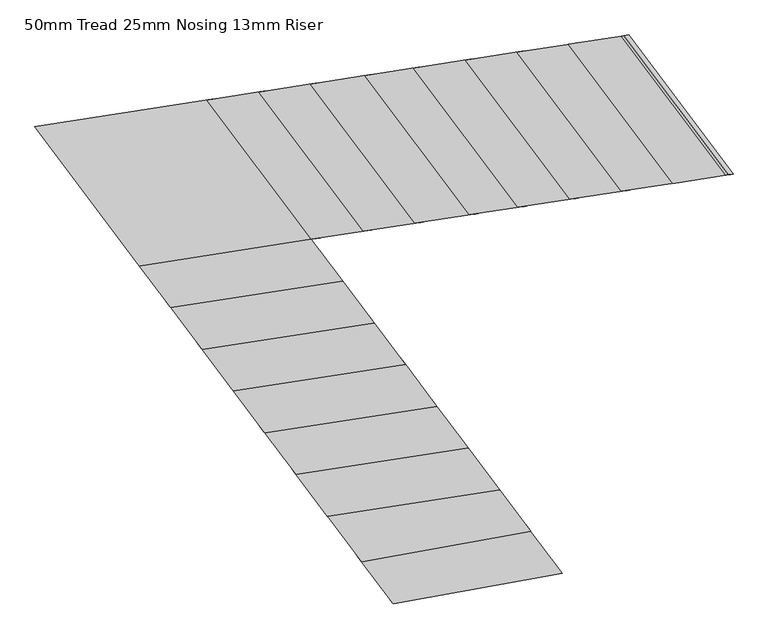
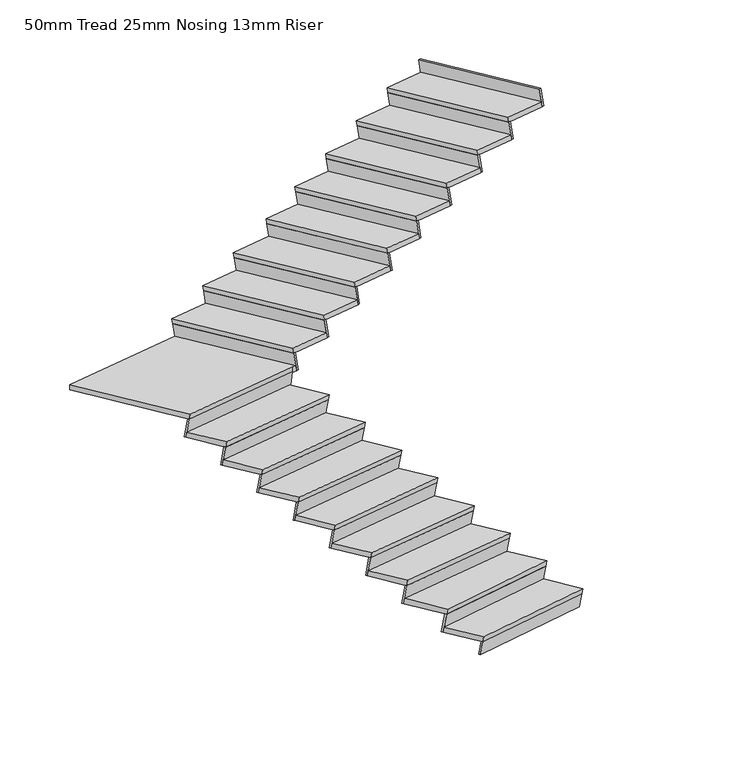
"""IFC4 building model written with IfcOpenShell, lengths in millimetres: stair flight geometry, 50mm Tread 25mm Nosing 13mm Riser."""

from ifc_helpers import new_model, si_unit, origin, place, context, project, spatial, faceted_brep, source, transform, mapped, element, save


def stair_flight_50mm_tread_25mm_nosing_13mm_riser_829bcf17(model_context):
    return source(origin(), model_context, "Body", "Brep", [
        faceted_brep([(80326.693796, 43447.2585725, 17175.0), (80321.8971276, 43453.651768, 17125.0), (79350.3599929, 43278.4852415, 17125.0), (79355.1566613, 43272.092046, 17175.0), (79551.9875613, 43009.747788, 17175.0), (80523.524696, 43184.9143144, 17175.0), (80518.7280276, 43191.3075099, 17125.0), (79547.1908928, 43016.1409835, 17125.0)], [[[0, 1, 2, 3]], [[3, 4, 5, 0]], [[2, 1, 6, 7]], [[4, 3, 2, 7]], [[0, 5, 6, 1]], [[5, 4, 7, 6]]]),
        faceted_brep([(80518.7280276, 43191.3075099, 17125.0), (80506.7363564, 43207.2904987, 17000.0), (80498.2569645, 43218.5921784, 17000.0), (80510.2486356, 43202.6091897, 17125.0), (79547.1908928, 43016.1409835, 17125.0), (79538.7115009, 43027.4426632, 17125.0), (79526.7198298, 43043.425652, 17000.0), (79535.1992217, 43032.1239722, 17000.0)], [[[0, 1, 2, 3]], [[4, 5, 6, 7]], [[1, 0, 4, 7]], [[2, 1, 7, 6]], [[3, 2, 6, 5]], [[0, 3, 5, 4]]]),
        faceted_brep([(80338.6854672, 43431.2755837, 17300.0), (80321.8971276, 43453.651768, 17125.0), (80313.4177356, 43464.9534477, 17125.0), (80330.2060752, 43442.5772635, 17300.0), (79367.1483324, 43256.1090573, 17300.0), (79358.6689405, 43267.410737, 17300.0), (79341.8806009, 43289.7869213, 17125.0), (79350.3599929, 43278.4852415, 17125.0)], [[[0, 1, 2, 3]], [[4, 5, 6, 7]], [[1, 0, 4, 7]], [[2, 1, 7, 6]], [[3, 2, 6, 5]], [[0, 3, 5, 4]]]),
        faceted_brep([(79158.1923254, 43534.614153, 17350.0), (79371.9450009, 43249.7158618, 17350.0), (80343.4821356, 43424.8823882, 17350.0), (80146.4335925, 43687.51673, 17350.0), (79153.3334732, 43541.0902296, 17300.0), (80141.5747402, 43693.9928066, 17300.0), (80338.6854672, 43431.2755837, 17300.0), (79367.1483324, 43256.1090573, 17300.0)], [[[0, 1, 2, 3]], [[4, 5, 6, 7]], [[1, 0, 4, 7]], [[3, 2, 6, 5]], [[3, 5, 4, 0]], [[2, 1, 7, 6]]]),
        faceted_brep([(80158.580723, 43671.3265386, 17475.0), (80141.5747402, 43693.9928066, 17300.0), (80132.9854219, 43705.4410008, 17300.0), (80149.9914046, 43682.7747328, 17475.0), (79170.3394559, 43518.4239616, 17475.0), (79161.7501375, 43529.8721558, 17475.0), (79144.7441548, 43552.5384238, 17300.0), (79153.3334732, 43541.0902296, 17300.0)], [[[0, 1, 2, 3]], [[4, 5, 6, 7]], [[1, 0, 4, 7]], [[2, 1, 7, 6]], [[3, 2, 6, 5]], [[0, 3, 5, 4]]]),
        faceted_brep([(78978.149765, 43774.5822268, 17525.0), (79175.1983081, 43511.947885, 17525.0), (80163.4395752, 43664.850462, 17525.0), (79966.3910321, 43927.4848038, 17525.0), (78973.2909128, 43781.0583034, 17475.0), (79961.5321798, 43933.9608804, 17475.0), (80158.580723, 43671.3265386, 17475.0), (79170.3394559, 43518.4239616, 17475.0)], [[[0, 1, 2, 3]], [[4, 5, 6, 7]], [[1, 0, 4, 7]], [[3, 2, 6, 5]], [[3, 5, 4, 0]], [[2, 1, 7, 6]]]),
        faceted_brep([(79978.5381626, 43911.2946124, 17650.0), (79961.5321798, 43933.9608804, 17475.0), (79952.9428615, 43945.4090746, 17475.0), (79969.9488442, 43922.7428066, 17650.0), (78990.2968955, 43758.3920354, 17650.0), (78981.7075771, 43769.8402296, 17650.0), (78964.7015944, 43792.5064976, 17475.0), (78973.2909128, 43781.0583034, 17475.0)], [[[0, 1, 2, 3]], [[4, 5, 6, 7]], [[1, 0, 4, 7]], [[2, 1, 7, 6]], [[3, 2, 6, 5]], [[0, 3, 5, 4]]]),
        faceted_brep([(78798.1072046, 44014.5503006, 17700.0), (78995.1557477, 43751.9159588, 17700.0), (79983.3970148, 43904.8185358, 17700.0), (79786.3484717, 44167.4528777, 17700.0), (78793.2483524, 44021.0263772, 17650.0), (79781.4896194, 44173.9289542, 17650.0), (79978.5381626, 43911.2946124, 17650.0), (78990.2968955, 43758.3920354, 17650.0)], [[[0, 1, 2, 3]], [[4, 5, 6, 7]], [[1, 0, 4, 7]], [[3, 2, 6, 5]], [[3, 5, 4, 0]], [[2, 1, 7, 6]]]),
        faceted_brep([(79798.4956022, 44151.2626862, 17825.0), (79781.4896194, 44173.9289542, 17650.0), (79772.9003011, 44185.3771484, 17650.0), (79789.9062838, 44162.7108804, 17825.0), (78810.2543351, 43998.3601092, 17825.0), (78801.6650168, 44009.8083034, 17825.0), (78784.659034, 44032.4745714, 17650.0), (78793.2483524, 44021.0263772, 17650.0)], [[[0, 1, 2, 3]], [[4, 5, 6, 7]], [[1, 0, 4, 7]], [[2, 1, 7, 6]], [[3, 2, 6, 5]], [[0, 3, 5, 4]]]),
        faceted_brep([(78618.0646442, 44254.5183745, 17875.0), (78815.1131873, 43991.8840326, 17875.0), (79803.3544544, 44144.7866096, 17875.0), (79606.3059113, 44407.4209515, 17875.0), (78613.205792, 44260.994451, 17825.0), (79601.447059, 44413.897028, 17825.0), (79798.4956022, 44151.2626862, 17825.0), (78810.2543351, 43998.3601092, 17825.0)], [[[0, 1, 2, 3]], [[4, 5, 6, 7]], [[1, 0, 4, 7]], [[3, 2, 6, 5]], [[3, 5, 4, 0]], [[2, 1, 7, 6]]]),
        faceted_brep([(79618.4530418, 44391.23076, 18000.0), (79601.447059, 44413.897028, 17825.0), (79592.8577407, 44425.3452222, 17825.0), (79609.8637234, 44402.6789542, 18000.0), (78630.2117747, 44238.328183, 18000.0), (78621.6224564, 44249.7763772, 18000.0), (78604.6164736, 44272.4426452, 17825.0), (78613.205792, 44260.994451, 17825.0)], [[[0, 1, 2, 3]], [[4, 5, 6, 7]], [[1, 0, 4, 7]], [[2, 1, 7, 6]], [[3, 2, 6, 5]], [[0, 3, 5, 4]]]),
        faceted_brep([(78438.0220838, 44494.4864483, 18050.0), (78635.0706269, 44231.8521065, 18050.0), (79623.311894, 44384.7546835, 18050.0), (79426.2633509, 44647.3890253, 18050.0), (78433.1632316, 44500.9625248, 18000.0), (79421.4044987, 44653.8651018, 18000.0), (79618.4530418, 44391.23076, 18000.0), (78630.2117747, 44238.328183, 18000.0)], [[[0, 1, 2, 3]], [[4, 5, 6, 7]], [[1, 0, 4, 7]], [[3, 2, 6, 5]], [[3, 5, 4, 0]], [[2, 1, 7, 6]]]),
        faceted_brep([(79438.4104814, 44631.1988338, 18175.0), (79421.4044987, 44653.8651018, 18000.0), (79412.8151803, 44665.313296, 18000.0), (79429.821163, 44642.647028, 18175.0), (78450.1692143, 44478.2962568, 18175.0), (78441.579896, 44489.744451, 18175.0), (78424.5739132, 44512.410719, 18000.0), (78433.1632316, 44500.9625248, 18000.0)], [[[0, 1, 2, 3]], [[4, 5, 6, 7]], [[1, 0, 4, 7]], [[2, 1, 7, 6]], [[3, 2, 6, 5]], [[0, 3, 5, 4]]]),
        faceted_brep([(78257.9795234, 44734.4545221, 18225.0), (78455.0280666, 44471.8201803, 18225.0), (79443.2693336, 44624.7227573, 18225.0), (79246.2207905, 44887.3570991, 18225.0), (78253.1206712, 44740.9305986, 18175.0), (79241.3619383, 44893.8331756, 18175.0), (79438.4104814, 44631.1988338, 18175.0), (78450.1692143, 44478.2962568, 18175.0)], [[[0, 1, 2, 3]], [[4, 5, 6, 7]], [[1, 0, 4, 7]], [[3, 2, 6, 5]], [[3, 5, 4, 0]], [[2, 1, 7, 6]]]),
        faceted_brep([(79258.367921, 44871.1669076, 18350.0), (79241.3619383, 44893.8331756, 18175.0), (79232.7726199, 44905.2813698, 18175.0), (79249.7786026, 44882.6151018, 18350.0), (78270.1266539, 44718.2643306, 18350.0), (78261.5373356, 44729.7125248, 18350.0), (78244.5313528, 44752.3787928, 18175.0), (78253.1206712, 44740.9305986, 18175.0)], [[[0, 1, 2, 3]], [[4, 5, 6, 7]], [[1, 0, 4, 7]], [[2, 1, 7, 6]], [[3, 2, 6, 5]], [[0, 3, 5, 4]]]),
        faceted_brep([(78077.936963, 44974.4225959, 18400.0), (78274.9855062, 44711.7882541, 18400.0), (79263.2267732, 44864.6908311, 18400.0), (79066.1782301, 45127.3251729, 18400.0), (78073.0781108, 44980.8986724, 18350.0), (79061.3193779, 45133.8012494, 18350.0), (79258.367921, 44871.1669076, 18350.0), (78270.1266539, 44718.2643306, 18350.0)], [[[0, 1, 2, 3]], [[4, 5, 6, 7]], [[1, 0, 4, 7]], [[3, 2, 6, 5]], [[3, 5, 4, 0]], [[2, 1, 7, 6]]]),
        faceted_brep([(79082.0920516, 45111.7177711, 18525.0), (79078.2694871, 45136.4238027, 18350.0), (79076.3388006, 45148.9022331, 18350.0), (79080.161365, 45124.1962014, 18525.0), (78090.0840935, 44958.2324044, 18525.0), (78081.4947752, 44969.6805986, 18525.0), (78064.4887924, 44992.3468666, 18350.0), (78073.0781108, 44980.8986724, 18350.0)], [[[0, 1, 2, 3]], [[4, 5, 6, 7]], [[1, 0, 4, 7]], [[2, 1, 7, 6]], [[3, 2, 6, 5]], [[0, 3, 5, 4]]]),
        faceted_brep([(78511.0457468, 45908.8852241, 18575.0), (77494.8010778, 45751.6499072, 18575.0), (78094.9429458, 44951.7563279, 18575.0), (79083.1842128, 45104.6589049, 18575.0), (79111.1876148, 45108.9916447, 18575.0), (78519.0467188, 45910.1231498, 18525.0), (79119.1885868, 45110.2295704, 18525.0), (79083.1842128, 45104.6589049, 18525.0), (79082.0920516, 45111.7177711, 18525.0), (78090.0840935, 44958.2324044, 18525.0), (77494.8010778, 45751.6499072, 18525.0)], [[[0, 1, 2, 3, 4]], [[5, 6, 7, 8, 9, 10]], [[1, 0, 5, 10]], [[2, 1, 10, 9]], [[4, 3, 7, 6]], [[4, 6, 5, 0]], [[3, 8, 7]], [[8, 3, 2, 9]]]),
        faceted_brep([(79091.1851848, 45105.8968305, 18700.0), (79119.1885868, 45110.2295704, 18525.0), (79133.3324406, 45112.4179345, 18525.0), (79105.3290387, 45108.0851946, 18700.0), (78491.0433168, 45905.7904099, 18700.0), (78505.1871707, 45907.978774, 18700.0), (78533.1905726, 45912.3115138, 18525.0), (78519.0467188, 45910.1231498, 18525.0)], [[[0, 1, 2, 3]], [[4, 5, 6, 7]], [[1, 0, 4, 7]], [[2, 1, 7, 6]], [[3, 2, 6, 5]], [[0, 3, 5, 4]]]),
        faceted_brep([(78807.5181269, 45954.7559972, 18750.0), (78483.0423448, 45904.5524842, 18750.0), (79083.1842128, 45104.6589049, 18750.0), (79407.6599949, 45154.8624178, 18750.0), (78815.5190989, 45955.9939229, 18700.0), (79415.6609669, 45156.1003435, 18700.0), (79091.1851848, 45105.8968305, 18700.0), (78491.0433168, 45905.7904099, 18700.0)], [[[0, 1, 2, 3]], [[4, 5, 6, 7]], [[1, 0, 4, 7]], [[3, 2, 6, 5]], [[3, 5, 4, 0]], [[2, 1, 7, 6]]]),
        faceted_brep([(79387.6575649, 45151.7676036, 18875.0), (79415.6609669, 45156.1003435, 18700.0), (79429.8048207, 45158.2887076, 18700.0), (79401.8014188, 45153.9559677, 18875.0), (78787.515697, 45951.661183, 18875.0), (78801.6595508, 45953.8495471, 18875.0), (78829.6629528, 45958.1822869, 18700.0), (78815.5190989, 45955.9939229, 18700.0)], [[[0, 1, 2, 3]], [[4, 5, 6, 7]], [[1, 0, 4, 7]], [[2, 1, 7, 6]], [[3, 2, 6, 5]], [[0, 3, 5, 4]]]),
        faceted_brep([(79103.990507, 46000.6267703, 18925.0), (78779.514725, 45950.4232573, 18925.0), (79379.656593, 45150.529678, 18925.0), (79704.132375, 45200.7331909, 18925.0), (79111.991479, 46001.864696, 18875.0), (79712.133347, 45201.9711166, 18875.0), (79387.6575649, 45151.7676036, 18875.0), (78787.515697, 45951.661183, 18875.0)], [[[0, 1, 2, 3]], [[4, 5, 6, 7]], [[1, 0, 4, 7]], [[3, 2, 6, 5]], [[3, 5, 4, 0]], [[2, 1, 7, 6]]]),
        faceted_brep([(79684.1299451, 45197.6383767, 19050.0), (79712.133347, 45201.9711166, 18875.0), (79726.2772009, 45204.1594807, 18875.0), (79698.2737989, 45199.8267408, 19050.0), (79083.9880771, 45997.5319561, 19050.0), (79098.1319309, 45999.7203202, 19050.0), (79126.1353329, 46004.05306, 18875.0), (79111.991479, 46001.864696, 18875.0)], [[[0, 1, 2, 3]], [[4, 5, 6, 7]], [[1, 0, 4, 7]], [[2, 1, 7, 6]], [[3, 2, 6, 5]], [[0, 3, 5, 4]]]),
        faceted_brep([(79418.5971144, 46049.3033057, 19100.0), (79075.9871051, 45996.2940304, 19100.0), (79676.1289731, 45196.4004511, 19100.0), (80018.7389824, 45249.4097263, 19100.0), (79426.5980864, 46050.5412313, 19050.0), (80026.7399544, 45250.647652, 19050.0), (79684.1299451, 45197.6383767, 19050.0), (79083.9880771, 45997.5319561, 19050.0)], [[[0, 1, 2, 3]], [[4, 5, 6, 7]], [[1, 0, 4, 7]], [[3, 2, 6, 5]], [[3, 5, 4, 0]], [[2, 1, 7, 6]]]),
        faceted_brep([(79998.7365524, 45246.3149121, 19225.0), (80026.7399544, 45250.647652, 19050.0), (80040.8838082, 45252.8360161, 19050.0), (80012.8804063, 45248.5032762, 19225.0), (79398.5946844, 46046.2084915, 19225.0), (79412.7385383, 46048.3968556, 19225.0), (79440.7419403, 46052.7295954, 19050.0), (79426.5980864, 46050.5412313, 19050.0)], [[[0, 1, 2, 3]], [[4, 5, 6, 7]], [[1, 0, 4, 7]], [[2, 1, 7, 6]], [[3, 2, 6, 5]], [[0, 3, 5, 4]]]),
        faceted_brep([(79696.9352673, 46092.3683165, 19275.0), (79390.5937125, 46044.9705658, 19275.0), (79990.7355805, 45245.0769865, 19275.0), (80297.0771353, 45292.4747371, 19275.0), (79704.9362393, 46093.6062422, 19225.0), (80305.0781072, 45293.7126628, 19225.0), (79998.7365524, 45246.3149121, 19225.0), (79398.5946844, 46046.2084915, 19225.0)], [[[0, 1, 2, 3]], [[4, 5, 6, 7]], [[1, 0, 4, 7]], [[3, 2, 6, 5]], [[3, 5, 4, 0]], [[2, 1, 7, 6]]]),
        faceted_brep([(80277.0747053, 45289.3799229, 19400.0), (80305.0781072, 45293.7126628, 19225.0), (80319.2219611, 45295.9010269, 19225.0), (80291.2185592, 45291.568287, 19400.0), (79676.9328373, 46089.2735023, 19400.0), (79691.0766912, 46091.4618664, 19400.0), (79719.0800931, 46095.7946062, 19225.0), (79704.9362393, 46093.6062422, 19225.0)], [[[0, 1, 2, 3]], [[4, 5, 6, 7]], [[1, 0, 4, 7]], [[2, 1, 7, 6]], [[3, 2, 6, 5]], [[0, 3, 5, 4]]]),
        faceted_brep([(79993.4076474, 46138.2390896, 19450.0), (79668.9318653, 46088.0355766, 19450.0), (80269.0737333, 45288.1419973, 19450.0), (80593.5495154, 45338.3455102, 19450.0), (80001.4086194, 46139.4770153, 19400.0), (80601.5504874, 45339.5834359, 19400.0), (80277.0747053, 45289.3799229, 19400.0), (79676.9328373, 46089.2735023, 19400.0)], [[[0, 1, 2, 3]], [[4, 5, 6, 7]], [[1, 0, 4, 7]], [[3, 2, 6, 5]], [[3, 5, 4, 0]], [[2, 1, 7, 6]]]),
        faceted_brep([(80573.5470854, 45335.250696, 19575.0), (80601.5504874, 45339.5834359, 19400.0), (80615.6943412, 45341.7718, 19400.0), (80587.6909393, 45337.4390601, 19575.0), (79973.4052174, 46135.1442754, 19575.0), (79987.5490713, 46137.3326395, 19575.0), (80015.5524732, 46141.6653793, 19400.0), (80001.4086194, 46139.4770153, 19400.0)], [[[0, 1, 2, 3]], [[4, 5, 6, 7]], [[1, 0, 4, 7]], [[2, 1, 7, 6]], [[3, 2, 6, 5]], [[0, 3, 5, 4]]]),
        faceted_brep([(80289.8800275, 46184.1098627, 19625.0), (79965.4042455, 46133.9063497, 19625.0), (80565.5461134, 45334.0127704, 19625.0), (80890.0218955, 45384.2162833, 19625.0), (80297.8809995, 46185.3477884, 19575.0), (80898.0228675, 45385.454209, 19575.0), (80573.5470854, 45335.250696, 19575.0), (79973.4052174, 46135.1442754, 19575.0)], [[[0, 1, 2, 3]], [[4, 5, 6, 7]], [[1, 0, 4, 7]], [[3, 2, 6, 5]], [[3, 5, 4, 0]], [[2, 1, 7, 6]]]),
        faceted_brep([(80870.0194655, 45381.1214692, 19750.0), (80898.0228675, 45385.454209, 19575.0), (80912.1667214, 45387.6425731, 19575.0), (80884.1633194, 45383.3098332, 19750.0), (80269.8775976, 46181.0150485, 19750.0), (80284.0214514, 46183.2034126, 19750.0), (80312.0248534, 46187.5361524, 19575.0), (80297.8809995, 46185.3477884, 19575.0)], [[[0, 1, 2, 3]], [[4, 5, 6, 7]], [[1, 0, 4, 7]], [[2, 1, 7, 6]], [[3, 2, 6, 5]], [[0, 3, 5, 4]]]),
        faceted_brep([(80586.3524076, 46229.9806358, 19800.0), (80261.8766256, 46179.7771228, 19800.0), (80862.0184936, 45379.8835435, 19800.0), (81186.4942756, 45430.0870564, 19800.0), (80594.3533796, 46231.2185615, 19750.0), (81194.4952476, 45431.3249821, 19750.0), (80870.0194655, 45381.1214692, 19750.0), (80269.8775976, 46181.0150485, 19750.0)], [[[0, 1, 2, 3]], [[4, 5, 6, 7]], [[1, 0, 4, 7]], [[3, 2, 6, 5]], [[3, 5, 4, 0]], [[2, 1, 7, 6]]]),
        faceted_brep([(81166.4918457, 45426.9922423, 19925.0), (81194.4952476, 45431.3249821, 19750.0), (81208.6391015, 45433.5133462, 19750.0), (81180.6356995, 45429.1806063, 19925.0), (80566.3499777, 46226.8858216, 19925.0), (80580.4938315, 46229.0741857, 19925.0), (80608.4972335, 46233.4069256, 19750.0), (80594.3533796, 46231.2185615, 19750.0)], [[[0, 1, 2, 3]], [[4, 5, 6, 7]], [[1, 0, 4, 7]], [[2, 1, 7, 6]], [[3, 2, 6, 5]], [[0, 3, 5, 4]]]),
        faceted_brep([(81462.9642258, 45472.8630154, 20100.0), (81490.9676277, 45477.1957552, 19925.0), (81505.1114816, 45479.3841193, 19925.0), (81477.1080797, 45475.0513794, 20100.0), (80862.8223578, 46272.7565947, 20100.0), (80876.9662117, 46274.9449588, 20100.0), (80904.9696136, 46279.2776987, 19925.0), (80890.8257597, 46277.0893346, 19925.0)], [[[0, 1, 2, 3]], [[4, 5, 6, 7]], [[1, 0, 4, 7]], [[2, 1, 7, 6]], [[3, 2, 6, 5]], [[0, 3, 5, 4]]]),
        faceted_brep([(80882.8247878, 46275.8514089, 19975.0), (80558.3490057, 46225.6478959, 19975.0), (81158.4908737, 45425.7543166, 19975.0), (81482.9666558, 45475.9578295, 19975.0), (80890.8257597, 46277.0893346, 19925.0), (81490.9676277, 45477.1957552, 19925.0), (81166.4918457, 45426.9922423, 19925.0), (80566.3499777, 46226.8858216, 19925.0)], [[[0, 1, 2, 3]], [[4, 5, 6, 7]], [[1, 0, 4, 7]], [[3, 2, 6, 5]], [[3, 5, 4, 0]], [[2, 1, 7, 6]]]),
    ])


if __name__ == "__main__":
    model = new_model("IFC4")
    model_context = context("Model", 3, world=origin())
    ifc_project = project(units=[si_unit("LENGTHUNIT", "METRE", prefix="MILLI")], contexts=[model_context])
    site = spatial("IfcSite", under=ifc_project)
    building = spatial("IfcBuilding", under=site)
    placement = place(None, origin())
    stair_flight_50mm_tread_25mm_nosing_13mm_riser_shape = stair_flight_50mm_tread_25mm_nosing_13mm_riser_829bcf17(model_context)
    element("IfcStairFlight", 1, ObjectType="50mm Tread 25mm Nosing 13mm Riser", at=placement, inside=building, context=model_context, shape_type="MappedRepresentation", body=[
        mapped(stair_flight_50mm_tread_25mm_nosing_13mm_riser_shape, transform((0.0, 0.0, 0.0), x_axis=(1.0, 0.0, 0.0), y_axis=(0.0, 1.0, 0.0), z_axis=(0.0, 0.0, 1.0))),
    ])
    save(model, "model.ifc")
